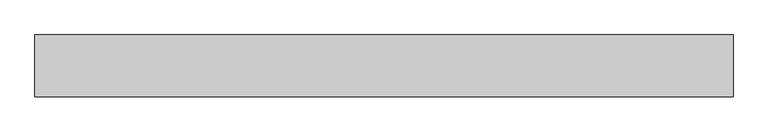
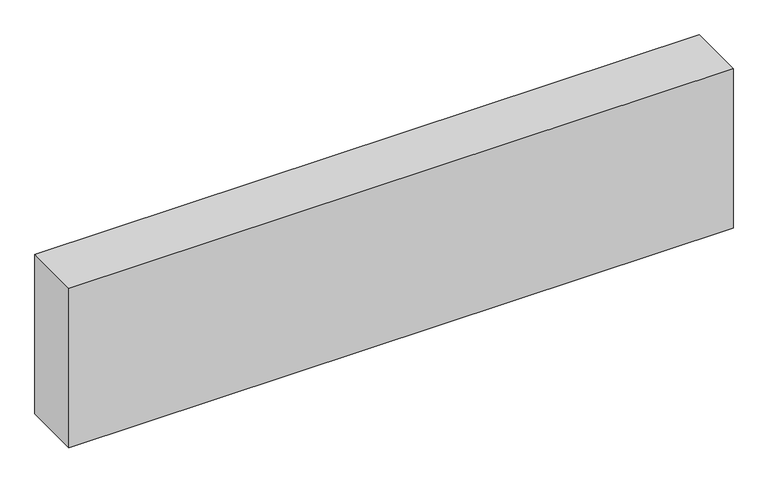
"""IFC4 building model written with IfcOpenShell, lengths in millimetres: proxy geometry, Structure006 588 : Structure006 588."""

from ifc_helpers import new_model, si_unit, frame, origin, place, context, project, spatial, polyline, outline, extrude, source, transform, mapped, element, save


def generic_models_a6ac43b1(model_context):
    return source(origin(), model_context, "Body", "SweptSolid", [
        extrude(outline(polyline([(3694.2883192, 10233.5750834), (3694.2883192, 10411.3750834), (5694.2883192, 10411.3750834), (5694.2883192, 10233.5750834), (3694.2883192, 10233.5750834)])), frame((0.0, 0.0, 39630.0976562), z_axis=(0.0, 0.0, 1.0), x_axis=(1.0, 0.0, 0.0)), (0.0, 0.0, 1.0), 508.0),
    ])


if __name__ == "__main__":
    model = new_model("IFC4")
    model_context = context("Model", 3, world=origin())
    ifc_project = project(units=[si_unit("LENGTHUNIT", "METRE", prefix="MILLI")], contexts=[model_context])
    site = spatial("IfcSite", under=ifc_project)
    building = spatial("IfcBuilding", under=site)
    placement = place(None, origin())
    generic_models_shape = generic_models_a6ac43b1(model_context)
    element("IfcBuildingElementProxy", 1, Name="Structure006 588 : Structure006 588", ObjectType="Structure006 588 : Structure006 588", at=placement, inside=building, context=model_context, shape_type="MappedRepresentation", body=[
        mapped(generic_models_shape, transform((0.0, 0.0, 0.0), x_axis=(1.0, 0.0, 0.0), y_axis=(0.0, 1.0, 0.0), z_axis=(0.0, 0.0, 1.0))),
    ])
    save(model, "model.ifc")

# Revit data of these elements
# Type "Structure006 588 : Structure006 588"
#   NameOverride = "Structure006"
# Element 1 (IfcBuildingElementProxy, "Structure006 588 : Structure006 588")
#   Materials on its faces: "STRUCTURAL MEMBER (SEE STRUCTURAL DWGS)"
# Materials
#   "STRUCTURAL MEMBER (SEE STRUCTURAL DWGS)": class "Unassigned", colour RGB 176 134 95, transparency 0, Cost = 0
